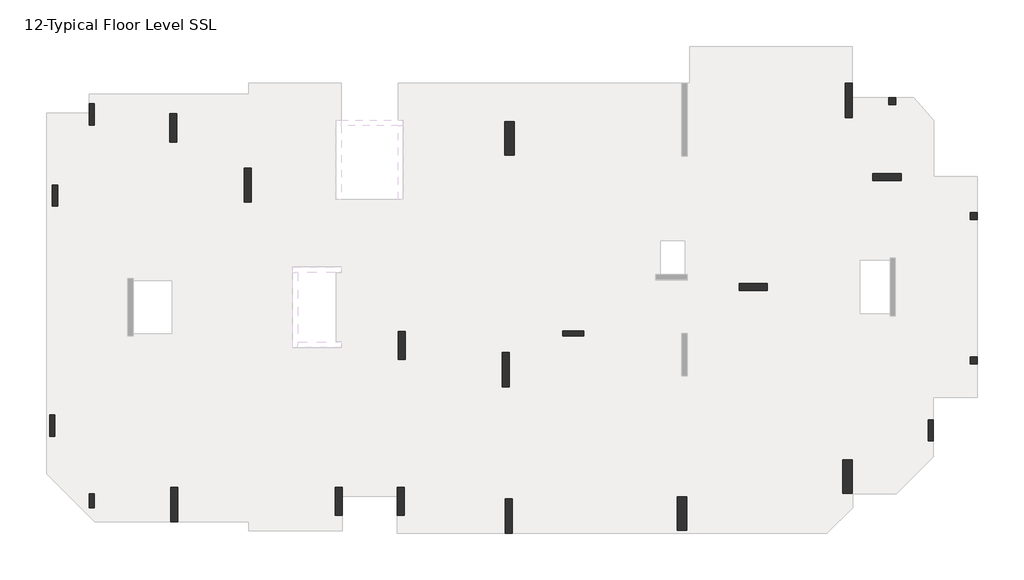
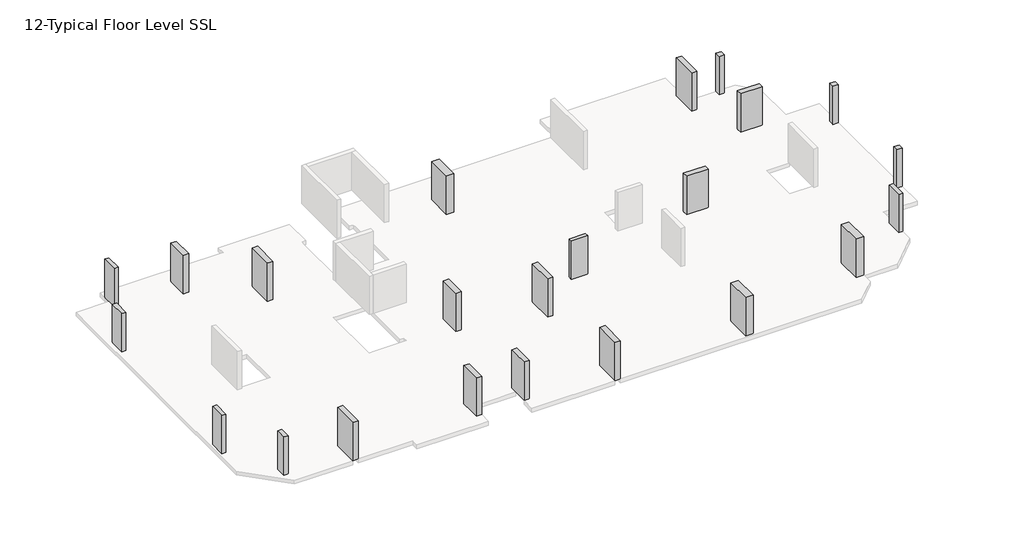
# One storey, part 2 of 2: 23 columns.
"""IFC4 building model written with IfcOpenShell, lengths in millimetres."""

from ifc_helpers import new_model, si_unit, origin, place, context, project, spatial, faceted_brep, element, save

model = new_model("IFC4")

# Units and contexts
model_context = context("Model", 3, world=origin())
ifc_project = project(units=[si_unit("LENGTHUNIT", "METRE", prefix="MILLI")], contexts=[model_context])

# Site, building, storey
site = spatial("IfcSite", under=ifc_project)
building = spatial("IfcBuilding", under=site)
storey = spatial("IfcBuildingStorey", under=building, Name="12-Typical Floor Level SSL", Elevation=30000.0)

# Columns
placement = place(None, origin())
element("IfcColumn", 1, ObjectType="M_Concrete-Rectangular-Column : C-1 (400 x 400mm)", at=placement, inside=storey, context=model_context, shape_type="Brep", body=[
    faceted_brep([(52549.9999998, 16712.0, 30000.0), (52549.9999998, 16312.0, 30000.0), (52149.9999998, 16312.0, 30000.0), (52149.9999998, 16712.0, 30000.0), (52549.9999998, 16712.0, 33000.0), (52549.9999998, 16312.0, 33000.0), (52549.9999998, 16312.0, 32700.0), (52549.9999998, 16712.0, 32700.0), (52149.9999998, 16312.0, 33000.0), (52149.9999998, 16312.0, 32700.0), (52149.9999998, 16712.0, 33000.0), (52149.9999998, 16712.0, 32700.0)], [[[0, 1, 2, 3]], [[4, 5, 6, 1, 0, 7]], [[5, 8, 9, 2, 1, 6]], [[8, 10, 11, 3, 2, 9]], [[10, 4, 7, 0, 3, 11]], [[4, 10, 8, 5]]]),
])
element("IfcColumn", 2, ObjectType="M_Concrete-Rectangular-Column : C-1 (400 x 400mm)", at=placement, inside=storey, context=model_context, shape_type="Brep", body=[
    faceted_brep([(47898.6337868, 23252.0, 30000.0), (47898.6337868, 22852.0, 30000.0), (47498.6337868, 22852.0, 30000.0), (47498.6337868, 23252.0, 30000.0), (47898.6337868, 23252.0, 33000.0), (47898.6337868, 22852.0, 33000.0), (47898.6337868, 22852.0, 32700.0), (47498.6337868, 22852.0, 33000.0), (47498.6337868, 22852.0, 32700.0), (47498.6337868, 23252.0, 33000.0)], [[[0, 1, 2, 3]], [[4, 5, 6, 1, 0]], [[5, 7, 8, 2, 1, 6]], [[7, 9, 3, 2, 8]], [[9, 4, 0, 3]], [[4, 9, 7, 5]]]),
])
element("IfcColumn", 3, ObjectType="M_Concrete-Rectangular-Column : C-1 (400 x 400mm)", at=placement, inside=storey, context=model_context, shape_type="Brep", body=[
    faceted_brep([(52549.9999998, 8504.0039609, 30000.0), (52549.9999998, 8104.0039609, 30000.0), (52149.9999998, 8104.0039609, 30000.0), (52149.9999998, 8504.0039609, 30000.0), (52549.9999998, 8504.0039609, 33000.0), (52549.9999998, 8104.0039609, 33000.0), (52549.9999998, 8104.0039609, 32700.0), (52549.9999998, 8504.0039609, 32700.0), (52149.9999998, 8104.0039609, 33000.0), (52149.9999998, 8104.0039609, 32700.0), (52149.9999998, 8504.0039609, 33000.0), (52149.9999998, 8504.0039609, 32700.0)], [[[0, 1, 2, 3]], [[4, 5, 6, 1, 0, 7]], [[5, 8, 9, 2, 1, 6]], [[8, 10, 11, 3, 2, 9]], [[10, 4, 7, 0, 3, 11]], [[4, 10, 8, 5]]]),
])
element("IfcColumn", 4, ObjectType="M_Concrete-Rectangular-Column : C-2 (300 x 800mm)", at=placement, inside=storey, context=model_context, shape_type="Brep", body=[
    faceted_brep([(2352.0, 728.0, 30000.0), (2352.0, -72.0, 30000.0), (2052.0, -72.0, 30000.0), (2052.0, 728.0, 30000.0), (2352.0, 728.0, 33000.0), (2352.0, -72.0, 33000.0), (2352.0, -72.0, 32700.0), (2352.0, 728.0, 32700.0), (2052.0, -72.0, 33000.0), (2052.0, -72.0, 32700.0), (2052.0, 728.0, 33000.0), (2052.0, 728.0, 32700.0)], [[[0, 1, 2, 3]], [[4, 5, 6, 1, 0, 7]], [[5, 8, 9, 2, 1, 6]], [[8, 10, 11, 3, 2, 9]], [[10, 4, 7, 0, 3, 11]], [[4, 10, 8, 5]]]),
])
element("IfcColumn", 5, ObjectType="M_Concrete-Rectangular-Column : C-3(300 x 1200mm)", at=placement, inside=storey, context=model_context, shape_type="Brep", body=[
    faceted_brep([(2352.0, 22908.0000656, 30000.0), (2352.0, 21708.0000656, 30000.0), (2052.0, 21708.0000656, 30000.0), (2052.0, 22908.0000656, 30000.0), (2352.0, 22908.0000656, 33000.0), (2352.0, 21708.0000656, 33000.0), (2352.0, 21708.0000656, 32700.0), (2352.0, 22908.0000656, 32700.0), (2052.0, 21708.0000656, 33000.0), (2052.0, 21708.0000656, 32700.0), (2052.0, 22380.0004589, 33000.0), (2052.0, 22908.0000656, 33000.0), (2052.0, 22908.0000656, 32700.0)], [[[0, 1, 2, 3]], [[4, 5, 6, 1, 0, 7]], [[5, 8, 9, 2, 1, 6]], [[8, 10, 11, 12, 3, 2, 9]], [[11, 4, 7, 0, 3, 12]], [[4, 11, 10, 8, 5]]]),
])
element("IfcColumn", 6, ObjectType="M_Concrete-Rectangular-Column : C-3(300 x 1200mm)", at=placement, inside=storey, context=model_context, shape_type="Brep", body=[
    faceted_brep([(257.9999999, 18288.0, 30000.0), (257.9999999, 17088.0, 30000.0), (-42.0000001, 17088.0, 30000.0), (-42.0000001, 18288.0, 30000.0), (257.9999999, 18288.0, 33000.0), (257.9999999, 17088.0, 33000.0), (257.9999999, 17088.0, 32700.0), (257.9999999, 18288.0, 32700.0), (-42.0000001, 17088.0, 33000.0), (-42.0000001, 17088.0, 32700.0), (-42.0000001, 18288.0, 33000.0), (-42.0000001, 18288.0, 32700.0)], [[[0, 1, 2, 3]], [[4, 5, 6, 1, 0, 7]], [[5, 8, 9, 2, 1, 6]], [[8, 10, 11, 3, 2, 9]], [[10, 4, 7, 0, 3, 11]], [[4, 10, 8, 5]]]),
])
element("IfcColumn", 7, ObjectType="M_Concrete-Rectangular-Column : C-3(300 x 1200mm)", at=placement, inside=storey, context=model_context, shape_type="Brep", body=[
    faceted_brep([(108.001803, 5201.9999858, 30000.0), (108.001803, 4001.9999858, 30000.0), (-191.998197, 4001.9999858, 30000.0), (-191.998197, 5201.9999858, 30000.0), (108.001803, 5201.9999858, 33000.0), (108.001803, 4001.9999858, 33000.0), (108.001803, 4001.9999858, 32700.0), (108.001803, 5201.9999858, 32700.0), (-191.998197, 4001.9999858, 33000.0), (-191.998197, 4001.9999858, 32700.0), (-191.998197, 5201.9999858, 33000.0), (-191.998197, 5201.9999858, 32700.0)], [[[0, 1, 2, 3]], [[4, 5, 6, 1, 0, 7]], [[5, 8, 9, 2, 1, 6]], [[8, 10, 11, 3, 2, 9]], [[10, 4, 7, 0, 3, 11]], [[4, 10, 8, 5]]]),
])
element("IfcColumn", 8, ObjectType="M_Concrete-Rectangular-Column : C-3(300 x 1200mm)", at=placement, inside=storey, context=model_context, shape_type="Brep", body=[
    faceted_brep([(50046.0009271, 4931.9999929, 30000.0), (50046.0009271, 3731.9999929, 30000.0), (49746.0009271, 3731.9999929, 30000.0), (49746.0009271, 4931.9999929, 30000.0), (50046.0009271, 4931.9999929, 33000.0), (50046.0009271, 3731.9999929, 33000.0), (50046.0009271, 3731.9999929, 32700.0), (50046.0009271, 4931.9999929, 32700.0), (49746.0009271, 3731.9999929, 33000.0), (49746.0009271, 3731.9999929, 32700.0), (49746.0009271, 4931.9999929, 33000.0), (49746.0009271, 4931.9999929, 32700.0)], [[[0, 1, 2, 3]], [[4, 5, 6, 1, 0, 7]], [[5, 8, 9, 2, 1, 6]], [[8, 10, 11, 3, 2, 9]], [[10, 4, 7, 0, 3, 11]], [[4, 10, 8, 5]]]),
])
element("IfcColumn", 9, ObjectType="M_Concrete-Rectangular-Column : C-3(300 x 1200mm)", at=placement, inside=storey, context=model_context, shape_type="Brep", body=[
    faceted_brep([(28975.9999998, 9996.0000019, 30000.0), (30175.9999998, 9996.0000019, 30000.0), (30175.9999998, 9696.0000019, 30000.0), (28975.9999998, 9696.0000019, 30000.0), (28975.9999998, 9996.0000019, 33000.0), (30175.9999998, 9996.0000019, 33000.0), (30175.9999998, 9996.0000019, 32700.0), (28975.9999998, 9996.0000019, 32700.0), (30175.9999998, 9696.0000019, 33000.0), (30175.9999998, 9696.0000019, 32700.0), (28975.9999998, 9696.0000019, 33000.0), (28975.9999998, 9696.0000019, 32700.0)], [[[0, 1, 2, 3]], [[4, 5, 6, 1, 0, 7]], [[5, 8, 9, 2, 1, 6]], [[8, 10, 11, 3, 2, 9]], [[10, 4, 7, 0, 3, 11]], [[4, 10, 8, 5]]]),
])
element("IfcColumn", 10, ObjectType="M_Concrete-Rectangular-Column : C-4 (400 x 1600mm)", at=placement, inside=storey, context=model_context, shape_type="Brep", body=[
    faceted_brep([(7021.9999999, 22340.0000078, 30000.0), (7021.9999999, 20740.0000078, 30000.0), (6621.9999999, 20740.0000078, 30000.0), (6621.9999999, 22340.0000078, 30000.0), (7021.9999999, 22340.0000078, 33000.0), (7021.9999999, 20740.0000078, 33000.0), (7021.9999999, 20740.0000078, 32700.0), (7021.9999999, 22340.0000078, 32700.0), (6621.9999999, 20740.0000078, 33000.0), (6621.9999999, 20740.0000078, 32700.0), (6621.9999999, 22340.0000078, 33000.0), (6621.9999999, 22340.0000078, 32700.0)], [[[0, 1, 2, 3]], [[4, 5, 6, 1, 0, 7]], [[5, 8, 9, 2, 1, 6]], [[8, 10, 11, 3, 2, 9]], [[10, 4, 7, 0, 3, 11]], [[4, 10, 8, 5]]]),
])
element("IfcColumn", 11, ObjectType="M_Concrete-Rectangular-Column : C-4 (400 x 1600mm)", at=placement, inside=storey, context=model_context, shape_type="Brep", body=[
    faceted_brep([(19969.9997488, 1087.9955348, 30000.0), (19969.9997488, -512.0044652, 30000.0), (19569.9997488, -512.0044652, 30000.0), (19569.9997488, 1087.9955348, 30000.0), (19969.9997488, 1087.9955348, 33000.0), (19969.9997488, -512.0044652, 33000.0), (19969.9997488, -512.0044652, 32700.0), (19969.9997488, 1087.9955348, 32700.0), (19569.9997488, -512.0044652, 33000.0), (19569.9997488, -512.0044652, 32700.0), (19569.9997488, 564.000519, 33000.0), (19569.9997488, 1087.9955348, 33000.0), (19569.9997488, 1087.9955348, 32700.0)], [[[0, 1, 2, 3]], [[4, 5, 6, 1, 0, 7]], [[5, 8, 9, 2, 1, 6]], [[8, 10, 11, 12, 3, 2, 9]], [[11, 4, 7, 0, 3, 12]], [[4, 11, 10, 8, 5]]]),
])
element("IfcColumn", 12, ObjectType="M_Concrete-Rectangular-Column : C-4 (400 x 1600mm)", at=placement, inside=storey, context=model_context, shape_type="Brep", body=[
    faceted_brep([(46605.9993605, 18950.0, 30000.0), (48205.9993605, 18950.0, 30000.0), (48205.9993605, 18550.0, 30000.0), (46605.9993605, 18550.0, 30000.0), (46605.9993605, 18950.0, 33000.0), (48205.9993605, 18950.0, 33000.0), (48205.9993605, 18950.0, 32700.0), (46605.9993605, 18950.0, 32700.0), (48205.9993605, 18550.0, 33000.0), (48205.9993605, 18550.0, 32700.0), (46605.9993605, 18550.0, 33000.0), (46605.9993605, 18550.0, 32700.0)], [[[0, 1, 2, 3]], [[4, 5, 6, 1, 0, 7]], [[5, 8, 9, 2, 1, 6]], [[8, 10, 11, 3, 2, 9]], [[10, 4, 7, 0, 3, 11]], [[4, 10, 8, 5]]]),
])
element("IfcColumn", 13, ObjectType="M_Concrete-Rectangular-Column : C-5 (400 x 1600mm)", at=placement, inside=storey, context=model_context, shape_type="Brep", body=[
    faceted_brep([(20030.000009, 9955.9999979, 30000.0), (20030.000009, 8355.9999979, 30000.0), (19630.000009, 8355.9999979, 30000.0), (19630.000009, 9955.9999979, 30000.0), (20030.000009, 9955.9999979, 33000.0), (20030.000009, 8355.9999979, 33000.0), (20030.000009, 8355.9999979, 32700.0), (20030.000009, 9955.9999979, 32700.0), (19630.000009, 8355.9999979, 33000.0), (19630.000009, 8355.9999979, 32700.0), (19630.000009, 9955.9999979, 33000.0), (19630.000009, 9955.9999979, 32700.0)], [[[0, 1, 2, 3]], [[4, 5, 6, 1, 0, 7]], [[5, 8, 9, 2, 1, 6]], [[8, 10, 11, 3, 2, 9]], [[10, 4, 7, 0, 3, 11]], [[4, 10, 8, 5]]]),
])
element("IfcColumn", 14, ObjectType="M_Concrete-Rectangular-Column : C-5 (400 x 1600mm)", at=placement, inside=storey, context=model_context, shape_type="Brep", body=[
    faceted_brep([(16429.9999981, 1088.0, 30000.0), (16429.9999981, -512.0, 30000.0), (16029.9999981, -512.0, 30000.0), (16029.9999981, 1088.0, 30000.0), (16429.9999981, 1088.0, 33000.0), (16429.9999981, 564.000519, 33000.0), (16429.9999981, -512.0, 33000.0), (16429.9999981, -512.0, 32700.0), (16429.9999981, 1088.0, 32700.0), (16029.9999981, -512.0, 33000.0), (16029.9999981, -512.0, 32700.0), (16029.9999981, 1088.0, 33000.0), (16029.9999981, 1088.0, 32700.0)], [[[0, 1, 2, 3]], [[4, 5, 6, 7, 1, 0, 8]], [[6, 9, 10, 2, 1, 7]], [[9, 11, 12, 3, 2, 10]], [[11, 4, 8, 0, 3, 12]], [[4, 11, 9, 6, 5]]]),
])
element("IfcColumn", 15, ObjectType="M_Concrete-Rectangular-Column : C-5 (400 x 1600mm)", at=placement, inside=storey, context=model_context, shape_type="Brep", body=[
    faceted_brep([(38998.0014887, 12692.0079212, 30000.0), (40598.0014887, 12692.0079212, 30000.0), (40598.0014887, 12292.0079212, 30000.0), (38998.0014887, 12292.0079212, 30000.0), (38998.0014887, 12692.0079212, 33000.0), (40598.0014887, 12692.0079212, 33000.0), (40598.0014887, 12692.0079212, 32700.0), (38998.0014887, 12692.0079212, 32700.0), (40598.0014887, 12292.0079212, 33000.0), (40598.0014887, 12292.0079212, 32700.0), (38998.0014887, 12292.0079212, 33000.0), (38998.0014887, 12292.0079212, 32700.0)], [[[0, 1, 2, 3]], [[4, 5, 6, 1, 0, 7]], [[5, 8, 9, 2, 1, 6]], [[8, 10, 11, 3, 2, 9]], [[10, 4, 7, 0, 3, 11]], [[4, 10, 8, 5]]]),
])
element("IfcColumn", 16, ObjectType="M_Concrete-Rectangular-Column : C-6 (400 x 1950mm)", at=placement, inside=storey, context=model_context, shape_type="Brep", body=[
    faceted_brep([(11270.0000427, 19262.9999996, 30000.0), (11270.0000427, 17312.9999996, 30000.0), (10870.0000427, 17312.9999996, 30000.0), (10870.0000427, 19262.9999996, 30000.0), (11270.0000427, 19262.9999996, 33000.0), (11270.0000427, 17312.9999996, 33000.0), (11270.0000427, 17312.9999996, 32700.0), (11270.0000427, 19262.9999996, 32700.0), (10870.0000427, 17312.9999996, 33000.0), (10870.0000427, 17312.9999996, 32700.0), (10870.0000427, 19262.9999996, 33000.0), (10870.0000427, 19262.9999996, 32700.0)], [[[0, 1, 2, 3]], [[4, 5, 6, 1, 0, 7]], [[5, 8, 9, 2, 1, 6]], [[8, 10, 11, 3, 2, 9]], [[10, 4, 7, 0, 3, 11]], [[4, 10, 8, 5]]]),
])
element("IfcColumn", 17, ObjectType="M_Concrete-Rectangular-Column : C-6 (400 x 1950mm)", at=placement, inside=storey, context=model_context, shape_type="Brep", body=[
    faceted_brep([(7082.0000416, 1083.0000153, 30000.0), (7082.0000416, -866.9999847, 30000.0), (6682.0000416, -866.9999847, 30000.0), (6682.0000416, 1083.0000153, 30000.0), (7082.0000416, 1083.0000153, 33000.0), (7082.0000416, -866.9999847, 33000.0), (7082.0000416, -866.9999847, 32700.0), (7082.0000416, 1083.0000153, 32700.0), (6682.0000416, -866.9999847, 33000.0), (6682.0000416, -866.9999847, 32700.0), (6682.0000416, 1083.0000153, 33000.0), (6682.0000416, 1083.0000153, 32700.0)], [[[0, 1, 2, 3]], [[4, 5, 6, 1, 0, 7]], [[5, 8, 9, 2, 1, 6]], [[8, 10, 11, 3, 2, 9]], [[10, 4, 7, 0, 3, 11]], [[4, 10, 8, 5]]]),
])
element("IfcColumn", 18, ObjectType="M_Concrete-Rectangular-Column : C-6 (400 x 1950mm)", at=placement, inside=storey, context=model_context, shape_type="Brep", body=[
    faceted_brep([(26113.9999998, 422.995535, 30000.0), (26113.9999998, -1527.004465, 30000.0), (25713.9999998, -1527.004465, 30000.0), (25713.9999998, 422.995535, 30000.0), (26113.9999998, 422.995535, 33000.0), (26113.9999998, -1527.004465, 33000.0), (26113.9999998, -1527.004465, 32700.0), (26113.9999998, 422.995535, 32700.0), (25713.9999998, -1527.004465, 33000.0), (25713.9999998, -1527.004465, 32700.0), (25713.9999998, 422.995535, 33000.0), (25713.9999998, 422.995535, 32700.0)], [[[0, 1, 2, 3]], [[4, 5, 6, 1, 0, 7]], [[5, 8, 9, 2, 1, 6]], [[8, 10, 11, 3, 2, 9]], [[10, 4, 7, 0, 3, 11]], [[4, 10, 8, 5]]]),
])
element("IfcColumn", 19, ObjectType="M_Concrete-Rectangular-Column : C-6 (400 x 1950mm)", at=placement, inside=storey, context=model_context, shape_type="Brep", body=[
    faceted_brep([(45446.0007483, 24087.0, 30000.0), (45446.0007483, 22137.0, 30000.0), (45046.0007483, 22137.0, 30000.0), (45046.0007483, 24087.0, 30000.0), (45446.0007483, 24087.0, 33000.0), (45446.0007483, 23252.0000315, 33000.0), (45446.0007483, 22137.0, 33000.0), (45446.0007483, 22137.0, 32700.0), (45446.0007483, 24087.0, 32700.0), (45046.0007483, 22137.0, 33000.0), (45046.0007483, 22137.0, 32700.0), (45046.0007483, 24087.0, 33000.0), (45046.0007483, 24087.0, 32700.0)], [[[0, 1, 2, 3]], [[4, 5, 6, 7, 1, 0, 8]], [[6, 9, 10, 2, 1, 7]], [[9, 11, 12, 3, 2, 10]], [[11, 4, 8, 0, 3, 12]], [[4, 11, 9, 6, 5]]]),
])
element("IfcColumn", 20, ObjectType="M_Concrete-Rectangular-Column : C-6 (400 x 1950mm)", at=placement, inside=storey, context=model_context, shape_type="Brep", body=[
    faceted_brep([(25934.0000455, 8751.0001824, 30000.0), (25934.0000455, 6801.0001824, 30000.0), (25534.0000455, 6801.0001824, 30000.0), (25534.0000455, 8751.0001824, 30000.0), (25934.0000455, 8751.0001824, 33000.0), (25934.0000455, 6801.0001824, 33000.0), (25934.0000455, 6801.0001824, 32700.0), (25934.0000455, 8751.0001824, 32700.0), (25534.0000455, 6801.0001824, 33000.0), (25534.0000455, 6801.0001824, 32700.0), (25534.0000455, 8751.0001824, 33000.0), (25534.0000455, 8751.0001824, 32700.0)], [[[0, 1, 2, 3]], [[4, 5, 6, 1, 0, 7]], [[5, 8, 9, 2, 1, 6]], [[8, 10, 11, 3, 2, 9]], [[10, 4, 7, 0, 3, 11]], [[4, 10, 8, 5]]]),
])
element("IfcColumn", 21, ObjectType="M_Concrete-Rectangular-Column : C-7 (550 x 1900mm)", at=placement, inside=storey, context=model_context, shape_type="Brep", body=[
    faceted_brep([(36035.9999998, 548.0007983, 30000.0), (36035.9999998, -1351.9992017, 30000.0), (35485.9999998, -1351.9992017, 30000.0), (35485.9999998, 548.0007983, 30000.0), (36035.9999998, 548.0007983, 33000.0), (36035.9999998, -1351.9992017, 33000.0), (36035.9999998, -1351.9992017, 32700.0), (36035.9999998, 548.0007983, 32700.0), (35485.9999998, -1351.9992017, 33000.0), (35485.9999998, -1351.9992017, 32700.0), (35485.9999998, 548.0007983, 33000.0), (35485.9999998, 548.0007983, 32700.0)], [[[0, 1, 2, 3]], [[4, 5, 6, 1, 0, 7]], [[5, 8, 9, 2, 1, 6]], [[8, 10, 11, 3, 2, 9]], [[10, 4, 7, 0, 3, 11]], [[4, 10, 8, 5]]]),
])
element("IfcColumn", 22, ObjectType="M_Concrete-Rectangular-Column : C-7 (550 x 1900mm)", at=placement, inside=storey, context=model_context, shape_type="Brep", body=[
    faceted_brep([(45443.9999998, 2648.0, 30000.0), (45443.9999998, 748.0, 30000.0), (44893.9999998, 748.0, 30000.0), (44893.9999998, 2648.0, 30000.0), (45443.9999998, 2648.0, 33000.0), (45443.9999998, 748.0, 33000.0), (45443.9999998, 748.0, 32700.0), (45443.9999998, 2648.0, 32700.0), (44893.9999998, 748.0, 33000.0), (44893.9999998, 748.0, 32700.0), (44893.9999998, 2648.0, 33000.0), (44893.9999998, 2648.0, 32700.0)], [[[0, 1, 2, 3]], [[4, 5, 6, 1, 0, 7]], [[5, 8, 9, 2, 1, 6]], [[8, 10, 11, 3, 2, 9]], [[10, 4, 7, 0, 3, 11]], [[4, 10, 8, 5]]]),
])
element("IfcColumn", 23, ObjectType="M_Concrete-Rectangular-Column : C-7 (550 x 1900mm)", at=placement, inside=storey, context=model_context, shape_type="Brep", body=[
    faceted_brep([(26218.9999998, 21900.0, 30000.0), (26218.9999998, 20000.0, 30000.0), (25668.9999998, 20000.0, 30000.0), (25668.9999998, 21900.0, 30000.0), (26218.9999998, 21900.0, 33000.0), (26218.9999998, 20000.0, 33000.0), (26218.9999998, 20000.0, 32700.0), (26218.9999998, 21900.0, 32700.0), (25668.9999998, 20000.0, 33000.0), (25668.9999998, 20000.0, 32700.0), (25668.9999998, 21900.0, 33000.0), (25668.9999998, 21900.0, 32700.0)], [[[0, 1, 2, 3]], [[4, 5, 6, 1, 0, 7]], [[5, 8, 9, 2, 1, 6]], [[8, 10, 11, 3, 2, 9]], [[10, 4, 7, 0, 3, 11]], [[4, 10, 8, 5]]]),
])

save(model, "model.ifc")

# Revit data of these elements
# Type "M_Concrete-Rectangular-Column : C-1 (400 x 400mm)"
#   Type Mark = "C01"
#   b = 400 mm
#   h = 400 mm
#   Structural Material [instance default] = Concrete, Cast-in-Place gray
# Type "M_Concrete-Rectangular-Column : C-2 (300 x 800mm)"
#   Type Mark = "C02"
#   b = 300 mm
#   h = 800 mm
#   Structural Material [instance default] = Concrete, Cast-in-Place gray
# Type "M_Concrete-Rectangular-Column : C-3(300 x 1200mm)"
#   Type Mark = "C03"
#   b = 300 mm
#   h = 1200 mm
#   Structural Material [instance default] = Concrete, Cast-in-Place gray
# Type "M_Concrete-Rectangular-Column : C-4 (400 x 1600mm)"
#   Type Mark = "C04"
#   b = 400 mm
#   h = 1600 mm
#   Structural Material [instance default] = Concrete, Cast-in-Place gray
# Type "M_Concrete-Rectangular-Column : C-5 (400 x 1600mm)"
#   Type Mark = "C05"
#   b = 400 mm
#   h = 1600 mm
#   Structural Material [instance default] = Concrete, Cast-in-Place gray
# Type "M_Concrete-Rectangular-Column : C-6 (400 x 1950mm)"
#   Type Mark = "C06"
#   b = 400 mm
#   h = 1950 mm
#   Structural Material [instance default] = Concrete, Cast-in-Place gray
# Type "M_Concrete-Rectangular-Column : C-7 (550 x 1900mm)"
#   Type Mark = "C07"
#   b = 550 mm
#   h = 1900 mm
#   Structural Material [instance default] = Concrete, Cast-in-Place gray
# Elements 1, 2, 3 (IfcColumn, "M_Concrete-Rectangular-Column : C-1 (400 x 400mm)")
#   Structural Material = Concrete-RC
#   Phase Created = New Construction
#   Materials on its faces: "Concrete-RC"
# Element 4 (IfcColumn, "M_Concrete-Rectangular-Column : C-2 (300 x 800mm)")
#   Structural Material = Concrete-RC
#   Phase Created = New Construction
#   Materials on its faces: "Concrete-RC"
# Elements 5, 6, 7, 8, 9 (IfcColumn, "M_Concrete-Rectangular-Column : C-3(300 x 1200mm)")
#   Structural Material = Concrete-RC
#   Phase Created = New Construction
#   Materials on its faces: "Concrete-RC"
# Elements 10, 11, 12 (IfcColumn, "M_Concrete-Rectangular-Column : C-4 (400 x 1600mm)")
#   Structural Material = Concrete-RC
#   Phase Created = New Construction
#   Materials on its faces: "Concrete-RC"
# Elements 13, 14, 15 (IfcColumn, "M_Concrete-Rectangular-Column : C-5 (400 x 1600mm)")
#   Structural Material = Concrete-RC
#   Phase Created = New Construction
#   Materials on its faces: "Concrete-RC"
# Elements 16, 17, 18, 19, 20 (IfcColumn, "M_Concrete-Rectangular-Column : C-6 (400 x 1950mm)")
#   Structural Material = Concrete-RC
#   Phase Created = New Construction
#   Materials on its faces: "Concrete-RC"
# Elements 21, 22, 23 (IfcColumn, "M_Concrete-Rectangular-Column : C-7 (550 x 1900mm)")
#   Structural Material = Concrete-RC
#   Phase Created = New Construction
#   Materials on its faces: "Concrete-RC"
# Materials
#   "Concrete, Cast-in-Place gray": class "Concrete", colour RGB 192 192 192, transparency 0, Description = "Cast-in-place concrete", Cost = 0
#   "Concrete-RC": class "Concrete", colour RGB 128 128 128, transparency 0, Description = "High strength concrete", Cost = 0
